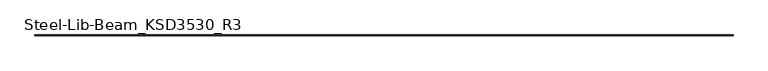
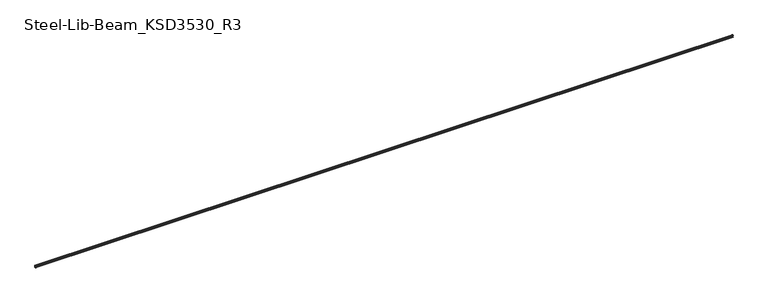
"""IFC4 building model written with IfcOpenShell, lengths in millimetres: beam geometry, Steel-Lib-Beam_KSD3530_R3 : BMS291_C-150×75x20x4.5."""

from ifc_helpers import new_model, si_unit, point, frame, frame_2d, origin, place, context, project, spatial, polyline, circle_curve, trimmed, segment, composite_curve, outline, extrude, source, transform, mapped, element, save


def steel_lib_beam_ksd3530_r3_7ad3471f(model_context):
    return source(origin(), model_context, "Body", "SweptSolid", [
        extrude(outline(composite_curve([segment(trimmed(circle_curve(frame_2d((-41.0, 66.0)), 9.0), [point((-50.0, 66.0))], [point((-41.0, 75.0))], False, "CARTESIAN"), True, "CONTINUOUS"), segment(polyline([(-41.0, 75.0), (16.0, 75.0)]), True, "CONTINUOUS"), segment(trimmed(circle_curve(frame_2d((16.0, 66.0)), 9.0), [point((16.0, 75.0))], [point((25.0, 66.0))], False, "CARTESIAN"), True, "CONTINUOUS"), segment(polyline([(25.0, 66.0), (25.0, -66.0)]), True, "CONTINUOUS"), segment(trimmed(circle_curve(frame_2d((16.0, -66.0)), 9.0), [point((25.0, -66.0))], [point((16.0, -75.0))], False, "CARTESIAN"), True, "CONTINUOUS"), segment(polyline([(16.0, -75.0), (-41.0, -75.0)]), True, "CONTINUOUS"), segment(trimmed(circle_curve(frame_2d((-41.0, -66.0)), 9.0), [point((-41.0, -75.0))], [point((-50.0, -66.0))], False, "CARTESIAN"), True, "CONTINUOUS"), segment(polyline([(-50.0, -66.0), (-50.0, -55.0), (-45.5, -55.0), (-45.5, -66.0)]), True, "CONTINUOUS"), segment(trimmed(circle_curve(frame_2d((-41.0, -66.0)), 4.5), [point((-45.5, -66.0))], [point((-41.0, -70.5))], True, "CARTESIAN"), True, "CONTINUOUS"), segment(polyline([(-41.0, -70.5), (16.0, -70.5)]), True, "CONTINUOUS"), segment(trimmed(circle_curve(frame_2d((16.0, -66.0)), 4.5), [point((16.0, -70.5))], [point((20.5, -66.0))], True, "CARTESIAN"), True, "CONTINUOUS"), segment(polyline([(20.5, -66.0), (20.5, 66.0)]), True, "CONTINUOUS"), segment(trimmed(circle_curve(frame_2d((16.0, 66.0)), 4.5), [point((20.5, 66.0))], [point((16.0, 70.5))], True, "CARTESIAN"), True, "CONTINUOUS"), segment(polyline([(16.0, 70.5), (-41.0, 70.5)]), True, "CONTINUOUS"), segment(trimmed(circle_curve(frame_2d((-41.0, 66.0)), 4.5), [point((-41.0, 70.5))], [point((-45.5, 66.0))], True, "CARTESIAN"), True, "CONTINUOUS"), segment(polyline([(-45.5, 66.0), (-45.5, 55.0), (-50.0, 55.0), (-50.0, 66.0)]), True, "CONTINUOUS")], self_intersect=False)), frame((-25632.5, 0.0, 0.0), z_axis=(1.0, 0.0, 0.0), x_axis=(0.0, 1.0, 0.0)), (0.0, 0.0, 1.0), 51265.0),
    ])


if __name__ == "__main__":
    model = new_model("IFC4")
    model_context = context("Model", 3, world=origin())
    ifc_project = project(units=[si_unit("LENGTHUNIT", "METRE", prefix="MILLI")], contexts=[model_context])
    site = spatial("IfcSite", under=ifc_project)
    building = spatial("IfcBuilding", under=site)
    placement = place(None, origin())
    steel_lib_beam_ksd3530_r3_shape = steel_lib_beam_ksd3530_r3_7ad3471f(model_context)
    element("IfcBeam", 1, ObjectType="Steel-Lib-Beam_KSD3530_R3 : BMS291_C-150×75x20x4.5", at=placement, inside=building, context=model_context, shape_type="MappedRepresentation", body=[
        mapped(steel_lib_beam_ksd3530_r3_shape, transform((0.0, 0.0, 0.0), x_axis=(1.0, 0.0, 0.0), y_axis=(0.0, 1.0, 0.0), z_axis=(0.0, 0.0, 1.0))),
    ])
    save(model, "model.ifc")

# Revit data of these elements
# Type "Steel-Lib-Beam_KSD3530_R3 : BMS291_C-150×75x20x4.5"
#   Keynote = "C-150×75x20x4.5"
#   SteelWeight = "Light"
#   x = 0.0250 m
#   t1 = 0.0090 m
#   t = 0.0045 m
#   Surface Area = 0.629834 m²/m
#   Section Area = 13.9688 cm²
#   Mass per Unit Length = 10.9655 kg/m
#   C = 0.0200 m
#   A = 0.0750 m
#   Length [instance default] = 1.5000 m
#   H = 0.1500 m
#   hec_material4 [instance default] = none
#   hec_material3 [instance default] = none
#   hec_material2 [instance default] = none
#   hec_material1 [instance default] = none
#   Structural Material [instance default] = Metal - Steel - Light Gauge
#   Assembly Code = ""
# Element 1 (IfcBeam, "Steel-Lib-Beam_KSD3530_R3 : BMS291_C-150×75x20x4.5")
#   Structural Material = none
# Materials
#   "Metal - Steel - Light Gauge": class "Metal", colour RGB 247 247 247, transparency 0
